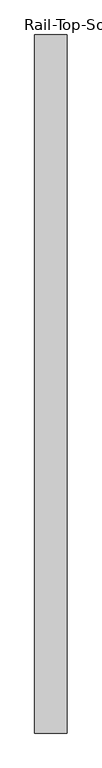
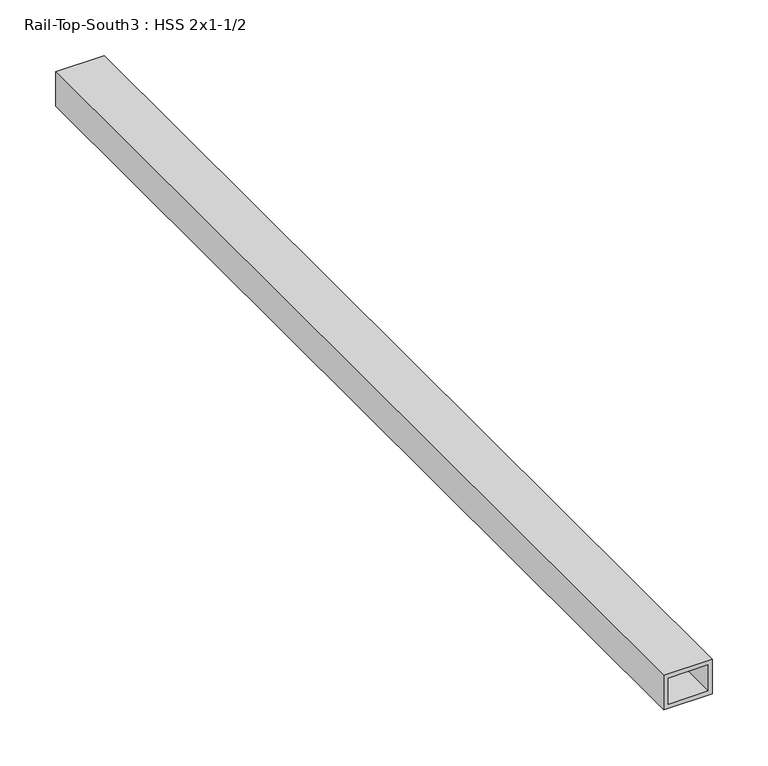
"""IFC4 building model written with IfcOpenShell, lengths in millimetres: proxy geometry, Rail-Top-South3 : HSS 2x1-1/2."""

from ifc_helpers import new_model, si_unit, frame, origin, place, context, project, spatial, polyline, outline, extrude, source, transform, mapped, element, save


def rail_top_south3_hss_2x1_1_2_6b80f164(model_context):
    return source(origin(), model_context, "Body", "SweptSolid", [
        extrude(outline(polyline([(2400.3, 587416.6934739), (2438.4, 587416.6934739), (2438.4, 587365.8934739), (2400.3, 587365.8934739), (2400.3, 587416.6934739)]), holes=[polyline([(2433.6375, 587411.9309739), (2405.0625, 587411.9309739), (2405.0625, 587370.6559739), (2433.6375, 587370.6559739), (2433.6375, 587411.9309739)])]), frame((0.0, -536301.7038841, 0.0), z_axis=(0.0, 1.0, 0.0), x_axis=(0.0, 0.0, 1.0)), (0.0, 0.0, 1.0), 1093.7875),
    ])


if __name__ == "__main__":
    model = new_model("IFC4")
    model_context = context("Model", 3, world=origin())
    ifc_project = project(units=[si_unit("LENGTHUNIT", "METRE", prefix="MILLI")], contexts=[model_context])
    site = spatial("IfcSite", under=ifc_project)
    building = spatial("IfcBuilding", under=site)
    placement = place(None, origin())
    rail_top_south3_hss_2x1_1_2_shape = rail_top_south3_hss_2x1_1_2_6b80f164(model_context)
    element("IfcBuildingElementProxy", 1, Name="Rail-Top-South3 : HSS 2x1-1/2", ObjectType="Rail-Top-South3 : HSS 2x1-1/2", at=placement, inside=building, context=model_context, shape_type="MappedRepresentation", body=[
        mapped(rail_top_south3_hss_2x1_1_2_shape, transform((0.0, 0.0, 0.0), x_axis=(1.0, 0.0, 0.0), y_axis=(0.0, 1.0, 0.0), z_axis=(0.0, 0.0, 1.0))),
    ])
    save(model, "model.ifc")

# Revit data of these elements
# Element 1 (IfcBuildingElementProxy, "Rail-Top-South3 : HSS 2x1-1/2")
#   Materials on its faces: "1-1/2\"X2\" GALV. STL HSS TUBING"
# Materials
#   "1-1/2\"X2\" GALV. STL HSS TUBING": class "Generic", colour RGB 211 211 207, transparency 0, Cost = 0
